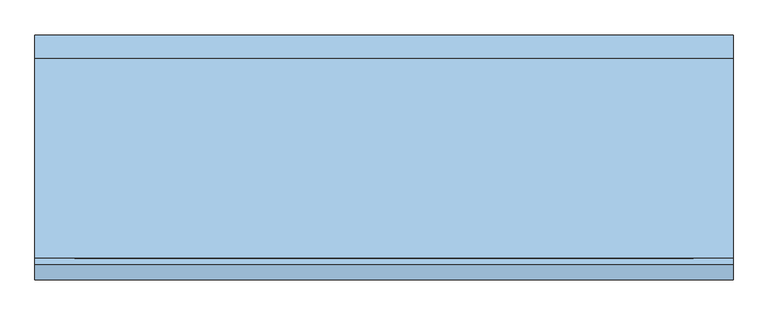
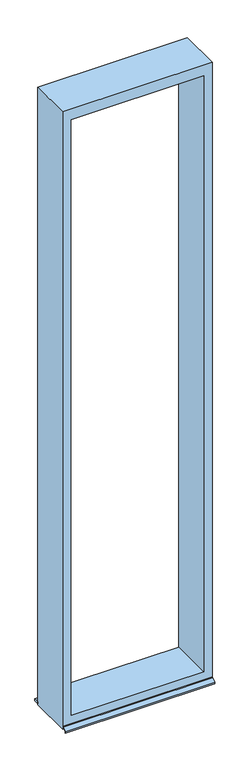
"""IFC4 building model written with IfcOpenShell, lengths in millimetres: window geometry, Fenster - Festverglasung : Feste Verglasung 4.58 x 1.03."""

from ifc_helpers import new_model, si_unit, frame, origin, place, context, project, spatial, polyline, outline, extrude, source, transform, mapped, element, save


def window_55cb6a76(model_context):
    return source(origin(), model_context, "Body", "SweptSolid", [
        extrude(outline(polyline([(5580.0, 525.0), (5580.0, -525.0), (1000.0, -525.0), (1000.0, 525.0), (5580.0, 525.0)]), holes=[polyline([(5500.0, 465.0), (1080.0, 465.0), (1080.0, -465.0), (5500.0, -465.0), (5500.0, 465.0)])]), frame((0.0, -151.5214598, 0.0), z_axis=(0.0, 1.0, 0.0), x_axis=(0.0, 0.0, 1.0)), (0.0, 0.0, 1.0), 300.0),
        extrude(outline(polyline([(-525.0, 184.0), (525.0, 184.0), (525.0, 148.4785402), (-525.0, 148.4785402), (-525.0, 184.0)])), frame((0.0, 0.0, 1005.0), z_axis=(0.0, 0.0, 1.0), x_axis=(1.0, 0.0, 0.0)), (0.0, 0.0, 1.0), 15.0),
        extrude(outline(polyline([(-161.5436142, 1020.0), (-151.5214598, 1020.0), (-151.5214598, 1018.0), (-161.3455321, 1018.0), (-182.0, 998.3604634), (-182.0, 990.0), (-184.0, 990.0), (-184.0, 1000.0), (-161.5436142, 1020.0)])), frame((-525.0, 0.0, 0.0), z_axis=(1.0, 0.0, 0.0), x_axis=(0.0, 1.0, 0.0)), (0.0, 0.0, 1.0), 1050.0),
    ])


if __name__ == "__main__":
    model = new_model("IFC4")
    model_context = context("Model", 3, world=origin())
    ifc_project = project(units=[si_unit("LENGTHUNIT", "METRE", prefix="MILLI")], contexts=[model_context])
    site = spatial("IfcSite", under=ifc_project)
    building = spatial("IfcBuilding", under=site)
    placement = place(None, origin())
    window_shape = window_55cb6a76(model_context)
    element("IfcWindow", 1, ObjectType="Fenster - Festverglasung : Feste Verglasung 4.58 x 1.03", at=placement, inside=building, context=model_context, shape_type="MappedRepresentation", body=[
        mapped(window_shape, transform((0.0, 0.0, 0.0), x_axis=(1.0, 0.0, 0.0), y_axis=(0.0, 1.0, 0.0), z_axis=(0.0, 0.0, 1.0))),
    ])
    save(model, "model.ifc")

# Revit data of these elements
# Type "Fenster - Festverglasung : Feste Verglasung 4.58 x 1.03"
#   Type Mark = "64"
#   Operation = "SinglePanel"
#   Keynote = "16.05.01"
#   Visual Light Transmittance = 0.9
#   Solar Heat Gain Coefficient = 0.78
#   Rough Width = 1.050 m
#   Rough Height = 4.580 m
#   Heat Transfer Coefficient (U) = 3.6886 W/(m²·K)
#   Rahmentiefe = 0.300 m
#   Rahmenhöhe unten = 0.080 m
#   Höhe oberer  Rahmen = 0.080 m
#   Rahmenbreite = 0.060 m
#   Height = 4.580 m
#   Einbautiefe (von außen) [instance default] = 0.080 m
#   Width = 1.050 m
#   Wall Closure = 3
#   Bild [instance default] = none
#   Glas [instance default] = none
#   Innere Fensterbank [instance default] = none
#   Äußere Fensterbank [instance default] = none
#   Construction Type Id = ""
#   Analytic Construction = (empty or 0)
# Element 1 (IfcWindow, "Fenster - Festverglasung : Feste Verglasung 4.58 x 1.03")
#   Einbautiefe (von außen) = 0.002479 m
#   Materials on its faces: "Kunststoff - Weiß", "Holz - Birke"
# Materials
#   "Kunststoff - Weiß": class "Kunststoff", colour RGB 249 249 249, transparency 0, Cost = 0
#   "Holz - Birke": class "Holz", colour RGB 213 164 103, transparency 0, Cost = 0
